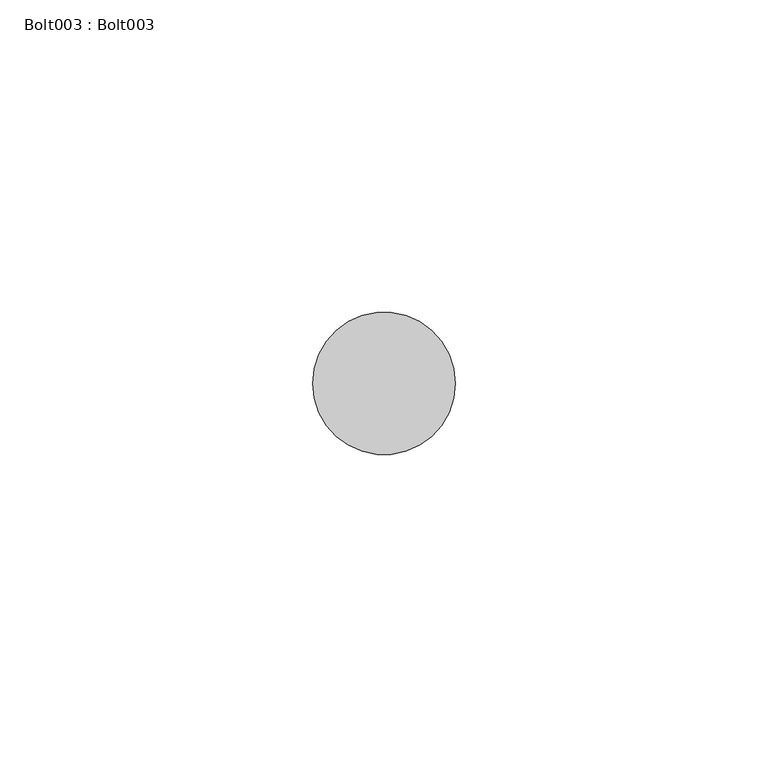
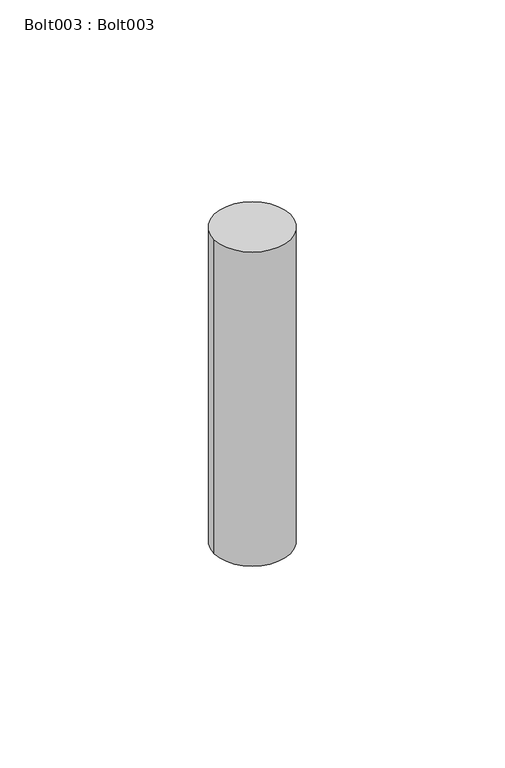
"""IFC4 building model written with IfcOpenShell, lengths in millimetres: proxy geometry, Bolt003 : Bolt003."""

from ifc_helpers import new_model, si_unit, point, frame, frame_2d, origin, place, context, project, spatial, circle_curve, trimmed, segment, composite_curve, outline, extrude, source, transform, mapped, element, save


def bolt003_bolt003_d269fbfb(model_context):
    return source(origin(), model_context, "Body", "SweptSolid", [
        extrude(outline(composite_curve([segment(trimmed(circle_curve(frame_2d((7415.2612305, -1781.8449707)), 11.4045168), [point((7403.8567137, -1781.8449707))], [point((7426.6657473, -1781.8449707))], False, "CARTESIAN"), True, "CONTINUOUS"), segment(trimmed(circle_curve(frame_2d((7415.2612305, -1781.8449707)), 11.4045168), [point((7426.6657473, -1781.8449707))], [point((7403.8567137, -1781.8449707))], False, "CARTESIAN"), True, "CONTINUOUS")], self_intersect=False)), frame((0.0, 0.0, 39994.0914664), z_axis=(0.0, 0.0, 1.0), x_axis=(1.0, 0.0, 0.0)), (0.0, 0.0, 1.0), 99.5545336),
    ])


if __name__ == "__main__":
    model = new_model("IFC4")
    model_context = context("Model", 3, world=origin())
    ifc_project = project(units=[si_unit("LENGTHUNIT", "METRE", prefix="MILLI")], contexts=[model_context])
    site = spatial("IfcSite", under=ifc_project)
    building = spatial("IfcBuilding", under=site)
    placement = place(None, origin())
    bolt003_bolt003_shape = bolt003_bolt003_d269fbfb(model_context)
    element("IfcBuildingElementProxy", 1, Name="Bolt003 : Bolt003", ObjectType="Bolt003 : Bolt003", at=placement, inside=building, context=model_context, shape_type="MappedRepresentation", body=[
        mapped(bolt003_bolt003_shape, transform((0.0, 0.0, 0.0), x_axis=(1.0, 0.0, 0.0), y_axis=(0.0, 1.0, 0.0), z_axis=(0.0, 0.0, 1.0))),
    ])
    save(model, "model.ifc")

# Revit data of these elements
# Type "Bolt003 : Bolt003"
#   NameOverride = "Bolt003"
# Element 1 (IfcBuildingElementProxy, "Bolt003 : Bolt003")
#   Materials on its faces: "BOLTS CONCEALED BY FLOOR FINISH"
# Materials
#   "BOLTS CONCEALED BY FLOOR FINISH": class "Unassigned", colour RGB 128 128 128, transparency 0
